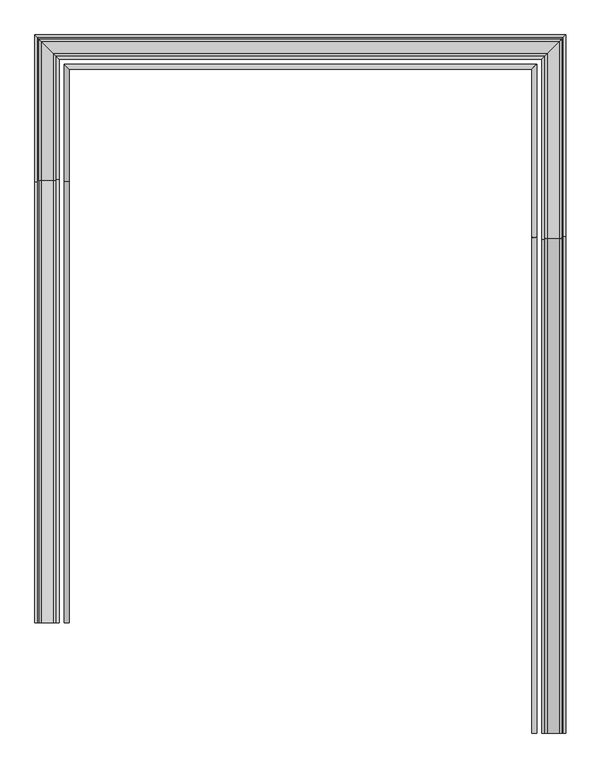
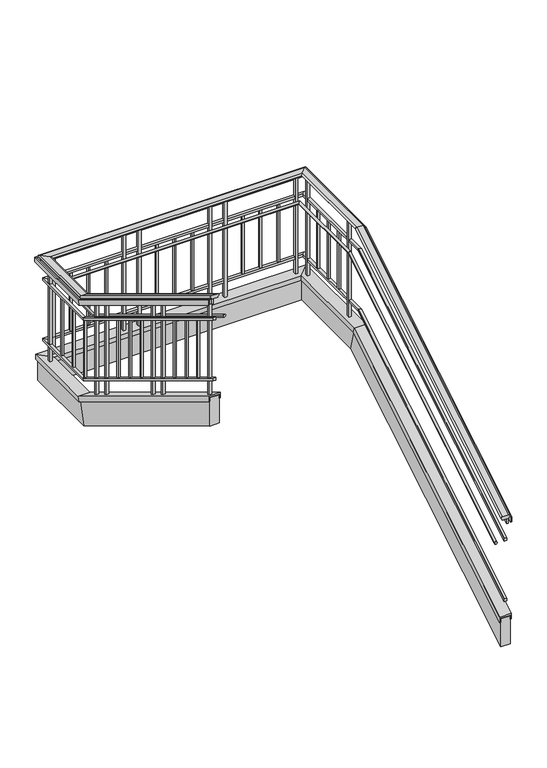
"""IFC4 building model written with IfcOpenShell, lengths in millimetres: railing geometry."""

from ifc_helpers import new_model, si_unit, frame, origin, place, context, project, spatial, polyline, ellipse_curve, outline, extrude, faceted_brep, source, transform, mapped, element, save
from ifc_brep_helpers import plane_surface, cylinder_surface, advanced_brep


def railing_cfa20eb0(model_context):
    return source(origin(), model_context, "Body", "SolidModel", [
        advanced_brep(
        [(-18297.9601205, -2131.266536, 1273.259246), (-18297.9601205, -2131.266536, 1247.2709218), (-18297.9601205, -2131.266536, 1236.1333333), (-18234.6103678, -2131.266536, 1236.1333333), (-18234.6103678, -2131.266536, 1247.1970062), (-18234.6103678, -2131.266536, 1273.259246), (-18297.9601205, 374.4632081, 2791.8833333), (-18297.9601205, 380.6724315, 2769.6581748), (-18297.9601205, 383.333464, 2760.1333333), (-18234.6103678, 383.333464, 2760.1333333), (-18234.6103678, 380.6900917, 2769.5949623), (-18234.6103678, 374.4632081, 2791.8833333), (-18297.9601205, 1312.1712113, 2791.8833333), (-18297.9601205, 1312.1712113, 2769.6581748), (-18297.9601205, 1312.1712113, 2760.1333333), (-18234.6103678, 1375.520964, 2760.1333333), (-18234.6103678, 1375.520964, 2769.5949623), (-18234.6103678, 1375.520964, 2791.8833333), (-20801.9121283, 1312.1712113, 2791.8833333), (-20801.9121283, 1312.1712113, 2769.6581748), (-20801.9121283, 1312.1712113, 2760.1333333), (-20865.2618809, 1375.520964, 2760.1333333), (-20865.2618809, 1375.520964, 2769.5949623), (-20865.2618809, 1375.520964, 2791.8833333), (-20801.9121283, 671.6037198, 2791.8833333), (-20801.9121283, 665.3944964, 2769.6581748), (-20801.9121283, 662.733464, 2760.1333333), (-20865.2618809, 662.733464, 2760.1333333), (-20865.2618809, 665.3768362, 2769.5949623), (-20865.2618809, 671.6037198, 2791.8833333), (-20801.9121283, -1572.466536, 4151.9259127), (-20865.2618809, -1572.466536, 4151.9259127), (-20865.2618809, -1572.466536, 4125.8636728), (-20865.2618809, -1572.466536, 4114.8), (-20801.9121283, -1572.466536, 4114.8), (-20801.9121283, -1572.466536, 4125.9375884)],
        [
            (0, 1, ellipse_curve(frame((-18297.9601205, -2131.266536, 1260.2650839), z_axis=(0.0, -1.0, 0.0), x_axis=(0.0, 0.0, -1.0)), 12.9941621, 11.1125793)),
            (1, 2),
            (2, 3),
            (3, 4),
            (4, 5, ellipse_curve(frame((-18234.6103678, -2131.266536, 1260.2281261), z_axis=(0.0, -1.0, 0.0), x_axis=(0.0, 0.0, -1.0)), 13.0311199, 11.1441855)),
            (5, 0),
            (0, 6),
            (6, 7, ellipse_curve(frame((-18297.9601205, 377.5678198, 2780.7707541), z_axis=(0.0, -0.9631193673564087, -0.26907449567543734), x_axis=(0.0, 0.2690744956754369, -0.9631193673564088)), 11.5381121, 11.1125793)),
            (7, 1),
            (7, 8),
            (8, 2),
            (8, 9),
            (9, 3),
            (9, 10),
            (10, 4),
            (10, 11, ellipse_curve(frame((-18234.6103678, 377.5766499, 2780.7391478), z_axis=(0.0, -0.9631193673564087, -0.26907449567543734), x_axis=(0.0, 0.2690744956754369, -0.9631193673564088)), 11.5709287, 11.1441855)),
            (11, 5),
            (11, 6),
            (6, 12),
            (12, 13, ellipse_curve(frame((-18297.9601205, 1312.1712113, 2780.7707541), z_axis=(0.7071067811865475, -0.7071067811865475, 0.0), x_axis=(-0.7071067811865474, -0.7071067811865476, 0.0)), 15.7155603, 11.1125793)),
            (13, 7),
            (13, 14),
            (14, 8),
            (14, 15),
            (15, 9),
            (15, 16),
            (16, 10),
            (16, 17, ellipse_curve(frame((-18234.6103678, 1375.520964, 2780.7391478), z_axis=(0.7071067811865475, -0.7071067811865475, 0.0), x_axis=(-0.7071067811865474, -0.7071067811865476, 0.0)), 15.7602583, 11.1441855)),
            (17, 11),
            (17, 12),
            (12, 18),
            (18, 19, ellipse_curve(frame((-20801.9121283, 1312.1712113, 2780.7707541), z_axis=(0.7071067811865475, 0.7071067811865475, 0.0), x_axis=(0.7071067811865476, -0.7071067811865474, 0.0)), 15.7155603, 11.1125793)),
            (19, 13),
            (19, 20),
            (20, 14),
            (20, 21),
            (21, 15),
            (21, 22),
            (22, 16),
            (22, 23, ellipse_curve(frame((-20865.2618809, 1375.520964, 2780.7391478), z_axis=(0.7071067811865475, 0.7071067811865475, 0.0), x_axis=(0.7071067811865476, -0.7071067811865474, 0.0)), 15.7602583, 11.1441855)),
            (23, 17),
            (23, 18),
            (18, 24),
            (24, 25, ellipse_curve(frame((-20801.9121283, 668.4991081, 2780.7707541), z_axis=(0.0, 0.9631193673564087, -0.2690744956754374), x_axis=(0.0, 0.26907449567543773, 0.9631193673564086)), 11.5381121, 11.1125793)),
            (25, 19),
            (25, 26),
            (26, 20),
            (26, 27),
            (27, 21),
            (27, 28),
            (28, 22),
            (28, 29, ellipse_curve(frame((-20865.2618809, 668.490278, 2780.7391478), z_axis=(0.0, 0.9631193673564087, -0.2690744956754374), x_axis=(0.0, 0.26907449567543773, 0.9631193673564086)), 11.5709287, 11.1441855)),
            (29, 23),
            (29, 24),
            (30, 31),
            (31, 32, ellipse_curve(frame((-20865.2618809, -1572.466536, 4138.8947927), z_axis=(0.0, -1.0, 0.0), x_axis=(0.0, 0.0, -1.0)), 13.0311199, 11.1441855)),
            (32, 33),
            (33, 34),
            (34, 35),
            (35, 30, ellipse_curve(frame((-20801.9121283, -1572.466536, 4138.9317505), z_axis=(0.0, -1.0, 0.0), x_axis=(0.0, 0.0, -1.0)), 12.9941621, 11.1125793)),
            (24, 30),
            (35, 25),
            (34, 26),
            (33, 27),
            (32, 28),
            (31, 29),
        ],
        [
            plane_surface(frame((-18266.3603678, -2131.266536, 1236.1333333), z_axis=(0.0, -1.0, 0.0), x_axis=(0.0, 0.0, 1.0))),
            cylinder_surface(frame((-18297.9601205, -2141.9629466, 1253.7824108), z_axis=(0.0, -0.8551978315540181, -0.518301716093344), x_axis=(1.0, 0.0, 0.0)), 11.1125793),
            plane_surface(frame((-18297.9601205, -2131.266536, 1247.2709218), z_axis=(-1.0000000000000002, 0.0, 0.0), x_axis=(0.0, 0.8551978315540182, 0.518301716093344))),
            plane_surface(frame((-18297.9601205, -2131.266536, 1236.1333333), z_axis=(0.0, 0.518301716093344, -0.8551978315540181), x_axis=(0.0, 0.8551978315540181, 0.518301716093344))),
            plane_surface(frame((-18234.6103678, -2131.266536, 1236.1333333), z_axis=(1.0, 0.0, 0.0), x_axis=(0.0, 0.8551978315540181, 0.518301716093344))),
            cylinder_surface(frame((-18234.6103678, -2141.9465651, 1253.7553812), z_axis=(0.0, -0.8551978315540181, -0.518301716093344), x_axis=(1.0, 0.0, 0.0)), 11.1441855),
            plane_surface(frame((-18234.6103678, -2131.266536, 1273.259246), z_axis=(0.0, -0.518301716093344, 0.8551978315540181), x_axis=(0.0, 0.8551978315540181, 0.518301716093344))),
            cylinder_surface(frame((-18297.9601205, 383.333464, 2780.7707541), z_axis=(0.0, -1.0, 0.0), x_axis=(1.0, 0.0, 0.0)), 11.1125793),
            plane_surface(frame((-18297.9601205, 380.6724315, 2769.6581748), z_axis=(-1.0, 0.0, 0.0), x_axis=(0.0, 1.0, 0.0))),
            plane_surface(frame((-18297.9601205, 383.333464, 2760.1333333), z_axis=(0.0, 0.0, -1.0), x_axis=(0.0, 1.0, 0.0))),
            plane_surface(frame((-18234.6103678, 383.333464, 2760.1333333), z_axis=(1.0, 0.0, 0.0), x_axis=(0.0, 1.0, 0.0))),
            cylinder_surface(frame((-18234.6103678, 383.333464, 2780.7391478), z_axis=(0.0, -1.0, 0.0), x_axis=(1.0, 0.0, 0.0)), 11.1441855),
            plane_surface(frame((-18234.6103678, 374.4632081, 2791.8833333), z_axis=(0.0, 0.0, 1.0), x_axis=(0.0, 1.0, 0.0))),
            cylinder_surface(frame((-18266.3603678, 1312.1712113, 2780.7707541), z_axis=(1.0, 0.0, 0.0), x_axis=(0.0, 1.0, 0.0)), 11.1125793),
            plane_surface(frame((-18297.9601205, 1312.1712113, 2769.6581748), z_axis=(0.0, -1.0, 0.0), x_axis=(-1.0, 0.0, 0.0))),
            plane_surface(frame((-18297.9601205, 1312.1712113, 2760.1333333), z_axis=(0.0, 0.0, -1.0), x_axis=(-1.0, 0.0, 0.0))),
            plane_surface(frame((-18234.6103678, 1375.520964, 2760.1333333), z_axis=(0.0, 1.0, 0.0), x_axis=(-1.0, 0.0, 0.0))),
            cylinder_surface(frame((-18266.3603678, 1375.520964, 2780.7391478), z_axis=(1.0, 0.0, 0.0), x_axis=(0.0, 1.0, 0.0)), 11.1441855),
            plane_surface(frame((-18234.6103678, 1375.520964, 2791.8833333), z_axis=(0.0, 0.0, 1.0), x_axis=(-1.0, 0.0, 0.0))),
            cylinder_surface(frame((-20801.9121283, 1343.770964, 2780.7707541), z_axis=(0.0, 1.0, 0.0), x_axis=(-1.0, 0.0, 0.0)), 11.1125793),
            plane_surface(frame((-20801.9121283, 1312.1712113, 2769.6581748), z_axis=(1.0, 0.0, 0.0), x_axis=(0.0, -1.0, 0.0))),
            plane_surface(frame((-20801.9121283, 1312.1712113, 2760.1333333), z_axis=(0.0, 0.0, -1.0), x_axis=(0.0, -1.0, 0.0))),
            plane_surface(frame((-20865.2618809, 1375.520964, 2760.1333333), z_axis=(-1.0, 0.0, 0.0), x_axis=(0.0, -1.0, 0.0))),
            cylinder_surface(frame((-20865.2618809, 1343.770964, 2780.7391478), z_axis=(0.0, 1.0, 0.0), x_axis=(-1.0, 0.0, 0.0)), 11.1441855),
            plane_surface(frame((-20865.2618809, 1375.520964, 2791.8833333), z_axis=(0.0, 0.0, 1.0), x_axis=(0.0, -1.0, 0.0))),
            plane_surface(frame((-20833.5118809, -1572.466536, 4114.8), z_axis=(0.0, -1.0, 0.0), x_axis=(0.0, 0.0, -1.0))),
            cylinder_surface(frame((-20801.9121283, 673.4298745, 2777.7824108), z_axis=(0.0, 0.855197831554018, -0.5183017160933441), x_axis=(-1.0, 0.0, 0.0)), 11.1125793),
            plane_surface(frame((-20801.9121283, 665.3944964, 2769.6581748), z_axis=(1.0, 0.0, 0.0), x_axis=(0.0, -0.8551978315540181, 0.5183017160933441))),
            plane_surface(frame((-20801.9121283, 662.733464, 2760.1333333), z_axis=(0.0, -0.5183017160933441, -0.855197831554018), x_axis=(0.0, -0.855197831554018, 0.5183017160933441))),
            plane_surface(frame((-20865.2618809, 662.733464, 2760.1333333), z_axis=(-1.0000000000000002, 0.0, 0.0), x_axis=(0.0, -0.8551978315540181, 0.5183017160933442))),
            cylinder_surface(frame((-20865.2618809, 673.413493, 2777.7553812), z_axis=(0.0, 0.855197831554018, -0.5183017160933441), x_axis=(-1.0, 0.0, 0.0)), 11.1441855),
            plane_surface(frame((-20865.2618809, 671.6037198, 2791.8833333), z_axis=(0.0, 0.5183017160933441, 0.8551978315540181), x_axis=(0.0, -0.8551978315540181, 0.5183017160933441))),
        ],
        [
            (0, [[1, 2, 3, 4, 5, 6]]),
            (1, [[-1, 7, 8, 9]]),
            (2, [[-2, -9, 10, 11]]),
            (3, [[-3, -11, 12, 13]]),
            (4, [[-4, -13, 14, 15]]),
            (5, [[-5, -15, 16, 17]]),
            (6, [[-6, -17, 18, -7]]),
            (7, [[-8, 19, 20, 21]]),
            (8, [[-10, -21, 22, 23]]),
            (9, [[-12, -23, 24, 25]]),
            (10, [[-14, -25, 26, 27]]),
            (11, [[-16, -27, 28, 29]]),
            (12, [[-18, -29, 30, -19]]),
            (13, [[-20, 31, 32, 33]]),
            (14, [[-22, -33, 34, 35]]),
            (15, [[-24, -35, 36, 37]]),
            (16, [[-26, -37, 38, 39]]),
            (17, [[-28, -39, 40, 41]]),
            (18, [[-30, -41, 42, -31]]),
            (19, [[-32, 43, 44, 45]]),
            (20, [[-34, -45, 46, 47]]),
            (21, [[-36, -47, 48, 49]]),
            (22, [[-38, -49, 50, 51]]),
            (23, [[-40, -51, 52, 53]]),
            (24, [[-42, -53, 54, -43]]),
            (25, [[55, 56, 57, 58, 59, 60]]),
            (26, [[-44, 61, -60, 62]]),
            (27, [[-46, -62, -59, 63]]),
            (28, [[-48, -63, -58, 64]]),
            (29, [[-50, -64, -57, 65]]),
            (30, [[-52, -65, -56, 66]]),
            (31, [[-54, -66, -55, -61]]),
        ],
    ),
        faceted_brep([(-18240.8852442, -2131.266536, 1236.1333333), (-18253.5852442, -2131.266536, 1236.1333333), (-18253.5852442, -2131.266536, 1184.1570556), (-18240.8852442, -2131.266536, 1184.1570556), (-18240.8852442, 383.333464, 2760.1333333), (-18253.5852442, 383.333464, 2760.1333333), (-18253.5852442, 395.7518222, 2715.6833333), (-18240.8852442, 395.7518222, 2715.6833333), (-18240.8852442, 1369.2460876, 2760.1333333), (-18253.5852442, 1356.5460876, 2760.1333333), (-18253.5852442, 1356.5460876, 2715.6833333), (-18240.8852442, 1369.2460876, 2715.6833333), (-20858.9870046, 1369.2460876, 2760.1333333), (-20846.2870046, 1356.5460876, 2760.1333333), (-20846.2870046, 1356.5460876, 2715.6833333), (-20858.9870046, 1369.2460876, 2715.6833333), (-20858.9870046, 662.733464, 2760.1333333), (-20846.2870046, 662.733464, 2760.1333333), (-20846.2870046, 650.3151057, 2715.6833333), (-20858.9870046, 650.3151057, 2715.6833333), (-20858.9870046, -1572.466536, 4114.8), (-20858.9870046, -1572.466536, 4062.8237223), (-20846.2870046, -1572.466536, 4062.8237223), (-20846.2870046, -1572.466536, 4114.8)], [[[0, 1, 2, 3]], [[1, 0, 4, 5]], [[2, 1, 5, 6]], [[3, 2, 6, 7]], [[0, 3, 7, 4]], [[5, 4, 8, 9]], [[6, 5, 9, 10]], [[7, 6, 10, 11]], [[4, 7, 11, 8]], [[9, 8, 12, 13]], [[10, 9, 13, 14]], [[11, 10, 14, 15]], [[8, 11, 15, 12]], [[13, 12, 16, 17]], [[14, 13, 17, 18]], [[15, 14, 18, 19]], [[12, 15, 19, 16]], [[20, 21, 22, 23]], [[17, 16, 20, 23]], [[18, 17, 23, 22]], [[19, 18, 22, 21]], [[16, 19, 21, 20]]]),
        faceted_brep([(-18202.7852442, -2131.266536, 1236.1333333), (-18215.4852442, -2131.266536, 1236.1333333), (-18215.4852442, -2131.266536, 1184.1570556), (-18202.7852442, -2131.266536, 1184.1570556), (-18202.7852442, 383.333464, 2760.1333333), (-18215.4852442, 383.333464, 2760.1333333), (-18215.4852442, 395.7518222, 2715.6833333), (-18202.7852442, 395.7518222, 2715.6833333), (-18202.7852442, 1407.3460876, 2760.1333333), (-18215.4852442, 1394.6460876, 2760.1333333), (-18215.4852442, 1394.6460876, 2715.6833333), (-18202.7852442, 1407.3460876, 2715.6833333), (-20897.0870046, 1407.3460876, 2760.1333333), (-20884.3870046, 1394.6460876, 2760.1333333), (-20884.3870046, 1394.6460876, 2715.6833333), (-20897.0870046, 1407.3460876, 2715.6833333), (-20897.0870046, 662.733464, 2760.1333333), (-20884.3870046, 662.733464, 2760.1333333), (-20884.3870046, 650.3151057, 2715.6833333), (-20897.0870046, 650.3151057, 2715.6833333), (-20897.0870046, -1572.466536, 4114.8), (-20897.0870046, -1572.466536, 4062.8237223), (-20884.3870046, -1572.466536, 4062.8237223), (-20884.3870046, -1572.466536, 4114.8)], [[[0, 1, 2, 3]], [[1, 0, 4, 5]], [[2, 1, 5, 6]], [[3, 2, 6, 7]], [[0, 3, 7, 4]], [[5, 4, 8, 9]], [[6, 5, 9, 10]], [[7, 6, 10, 11]], [[4, 7, 11, 8]], [[9, 8, 12, 13]], [[10, 9, 13, 14]], [[11, 10, 14, 15]], [[8, 11, 15, 12]], [[13, 12, 16, 17]], [[14, 13, 17, 18]], [[15, 14, 18, 19]], [[12, 15, 19, 16]], [[20, 21, 22, 23]], [[17, 16, 20, 23]], [[18, 17, 23, 22]], [[19, 18, 22, 21]], [[16, 19, 21, 20]]]),
        faceted_brep([(-18253.6603678, -2131.266536, 1037.2340635), (-18279.0603678, -2131.266536, 1037.2340635), (-18279.0603678, -2131.266536, 1007.5333333), (-18253.6603678, -2131.266536, 1007.5333333), (-18253.6603678, 376.2372592, 2556.9333333), (-18279.0603678, 376.2372592, 2556.9333333), (-18279.0603678, 383.333464, 2531.5333333), (-18253.6603678, 383.333464, 2531.5333333), (-18253.6603678, 1356.470964, 2556.9333333), (-18279.0603678, 1331.070964, 2556.9333333), (-18279.0603678, 1331.070964, 2531.5333333), (-18253.6603678, 1356.470964, 2531.5333333), (-20846.2118809, 1356.470964, 2556.9333333), (-20820.8118809, 1331.070964, 2556.9333333), (-20820.8118809, 1331.070964, 2531.5333333), (-20846.2118809, 1356.470964, 2531.5333333), (-20846.2118809, 669.8296687, 2556.9333333), (-20820.8118809, 669.8296687, 2556.9333333), (-20820.8118809, 662.733464, 2531.5333333), (-20846.2118809, 662.733464, 2531.5333333), (-20846.2118809, -1572.466536, 3915.9007301), (-20846.2118809, -1572.466536, 3886.2), (-20820.8118809, -1572.466536, 3886.2), (-20820.8118809, -1572.466536, 3915.9007301)], [[[0, 1, 2, 3]], [[1, 0, 4, 5]], [[2, 1, 5, 6]], [[3, 2, 6, 7]], [[0, 3, 7, 4]], [[5, 4, 8, 9]], [[6, 5, 9, 10]], [[7, 6, 10, 11]], [[4, 7, 11, 8]], [[9, 8, 12, 13]], [[10, 9, 13, 14]], [[11, 10, 14, 15]], [[8, 11, 15, 12]], [[13, 12, 16, 17]], [[14, 13, 17, 18]], [[15, 14, 18, 19]], [[12, 15, 19, 16]], [[20, 21, 22, 23]], [[17, 16, 20, 23]], [[18, 17, 23, 22]], [[19, 18, 22, 21]], [[16, 19, 21, 20]]]),
        advanced_brep(
        [(-18375.8978678, -2131.266536, 1020.2333333), (-18350.4978678, -2131.266536, 1020.2333333), (-18375.8978678, 383.333464, 2544.2333333), (-18350.4978678, 383.333464, 2544.2333333), (-18375.8978678, 1234.233464, 2544.2333333), (-18350.4978678, 1259.633464, 2544.2333333), (-20723.9743809, 1234.233464, 2544.2333333), (-20749.3743809, 1259.633464, 2544.2333333), (-20723.9743809, 662.733464, 2544.2333333), (-20749.3743809, 662.733464, 2544.2333333), (-20723.9743809, -1572.466536, 3898.9), (-20749.3743809, -1572.466536, 3898.9)],
        [
            (0, 1, ellipse_curve(frame((-18363.1978678, -2131.266536, 1020.2333333), z_axis=(0.0, -1.0, 0.0), x_axis=(0.0, 0.0, -1.0)), 14.8503651, 12.7)),
            (1, 0, ellipse_curve(frame((-18363.1978678, -2131.266536, 1020.2333333), z_axis=(0.0, -1.0, 0.0), x_axis=(0.0, 0.0, -1.0)), 14.8503651, 12.7)),
            (0, 2),
            (2, 3, ellipse_curve(frame((-18363.1978678, 383.333464, 2544.2333333), z_axis=(0.0, -0.9631193673564087, -0.2690744956754374), x_axis=(0.0, 0.2690744956754374, -0.9631193673564086)), 13.1863198, 12.7)),
            (3, 1),
            (3, 2, ellipse_curve(frame((-18363.1978678, 383.333464, 2544.2333333), z_axis=(0.0, -0.9631193673564087, -0.2690744956754374), x_axis=(0.0, 0.2690744956754374, -0.9631193673564086)), 13.1863198, 12.7)),
            (2, 4),
            (4, 5, ellipse_curve(frame((-18363.1978678, 1246.933464, 2544.2333333), z_axis=(0.7071067811865475, -0.7071067811865475, 0.0), x_axis=(-0.7071067811865474, -0.7071067811865476, 0.0)), 17.9605122, 12.7)),
            (5, 3),
            (5, 4, ellipse_curve(frame((-18363.1978678, 1246.933464, 2544.2333333), z_axis=(0.7071067811865475, -0.7071067811865475, 0.0), x_axis=(-0.7071067811865474, -0.7071067811865476, 0.0)), 17.9605122, 12.7)),
            (4, 6),
            (6, 7, ellipse_curve(frame((-20736.6743809, 1246.933464, 2544.2333333), z_axis=(0.7071067811865475, 0.7071067811865475, 0.0), x_axis=(0.7071067811865476, -0.7071067811865474, 0.0)), 17.9605122, 12.7)),
            (7, 5),
            (7, 6, ellipse_curve(frame((-20736.6743809, 1246.933464, 2544.2333333), z_axis=(0.7071067811865475, 0.7071067811865475, 0.0), x_axis=(0.7071067811865476, -0.7071067811865474, 0.0)), 17.9605122, 12.7)),
            (6, 8),
            (8, 9, ellipse_curve(frame((-20736.6743809, 662.733464, 2544.2333333), z_axis=(0.0, 0.9631193673564087, -0.26907449567543756), x_axis=(0.0, 0.26907449567543773, 0.9631193673564087)), 13.1863198, 12.7)),
            (9, 7),
            (9, 8, ellipse_curve(frame((-20736.6743809, 662.733464, 2544.2333333), z_axis=(0.0, 0.9631193673564087, -0.26907449567543756), x_axis=(0.0, 0.26907449567543773, 0.9631193673564087)), 13.1863198, 12.7)),
            (10, 11, ellipse_curve(frame((-20736.6743809, -1572.466536, 3898.9), z_axis=(0.0, -1.0, 0.0), x_axis=(0.0, 0.0, -1.0)), 14.8503651, 12.7)),
            (11, 10, ellipse_curve(frame((-20736.6743809, -1572.466536, 3898.9), z_axis=(0.0, -1.0, 0.0), x_axis=(0.0, 0.0, -1.0)), 14.8503651, 12.7)),
            (8, 10),
            (11, 9),
        ],
        [
            plane_surface(frame((-18363.1978678, -2131.266536, 1020.2333333), z_axis=(0.0, -1.0, 0.0), x_axis=(0.0, 0.0, 1.0))),
            cylinder_surface(frame((-18363.1978678, -2131.266536, 1020.2333333), z_axis=(0.0, -0.8551978315540182, -0.518301716093344), x_axis=(1.0, 0.0, 0.0)), 12.7),
            cylinder_surface(frame((-18363.1978678, 383.333464, 2544.2333333), z_axis=(0.0, -1.0, 0.0), x_axis=(1.0, 0.0, 0.0)), 12.7),
            cylinder_surface(frame((-18363.1978678, 1246.933464, 2544.2333333), z_axis=(1.0, 0.0, 0.0), x_axis=(0.0, 1.0, 0.0)), 12.7),
            cylinder_surface(frame((-20736.6743809, 1246.933464, 2544.2333333), z_axis=(0.0, 1.0, 0.0), x_axis=(-1.0, 0.0, 0.0)), 12.7),
            plane_surface(frame((-20736.6743809, -1572.466536, 3898.9), z_axis=(0.0, -1.0, 0.0), x_axis=(0.0, 0.0, -1.0))),
            cylinder_surface(frame((-20736.6743809, 662.733464, 2544.2333333), z_axis=(0.0, 0.855197831554018, -0.5183017160933443), x_axis=(-1.0, 0.0, 0.0)), 12.7),
        ],
        [
            (0, [[1, 2]]),
            (1, [[-1, 3, 4, 5]]),
            (1, [[-2, -5, 6, -3]]),
            (2, [[-4, 7, 8, 9]]),
            (2, [[-6, -9, 10, -7]]),
            (3, [[-8, 11, 12, 13]]),
            (3, [[-10, -13, 14, -11]]),
            (4, [[-12, 15, 16, 17]]),
            (4, [[-14, -17, 18, -15]]),
            (5, [[19, 20]]),
            (6, [[-16, 21, -20, 22]]),
            (6, [[-18, -22, -19, -21]]),
        ],
    ),
        faceted_brep([(-18253.6603678, -2131.266536, 402.2340635), (-18279.0603678, -2131.266536, 402.2340635), (-18279.0603678, -2131.266536, 372.5333333), (-18253.6603678, -2131.266536, 372.5333333), (-18253.6603678, 376.2372592, 1921.9333333), (-18279.0603678, 376.2372592, 1921.9333333), (-18279.0603678, 383.333464, 1896.5333333), (-18253.6603678, 383.333464, 1896.5333333), (-18253.6603678, 1356.470964, 1921.9333333), (-18279.0603678, 1331.070964, 1921.9333333), (-18279.0603678, 1331.070964, 1896.5333333), (-18253.6603678, 1356.470964, 1896.5333333), (-20846.2118809, 1356.470964, 1921.9333333), (-20820.8118809, 1331.070964, 1921.9333333), (-20820.8118809, 1331.070964, 1896.5333333), (-20846.2118809, 1356.470964, 1896.5333333), (-20846.2118809, 669.8296687, 1921.9333333), (-20820.8118809, 669.8296687, 1921.9333333), (-20820.8118809, 662.733464, 1896.5333333), (-20846.2118809, 662.733464, 1896.5333333), (-20846.2118809, -1572.466536, 3280.9007301), (-20846.2118809, -1572.466536, 3251.2), (-20820.8118809, -1572.466536, 3251.2), (-20820.8118809, -1572.466536, 3280.9007301)], [[[0, 1, 2, 3]], [[1, 0, 4, 5]], [[2, 1, 5, 6]], [[3, 2, 6, 7]], [[0, 3, 7, 4]], [[5, 4, 8, 9]], [[6, 5, 9, 10]], [[7, 6, 10, 11]], [[4, 7, 11, 8]], [[9, 8, 12, 13]], [[10, 9, 13, 14]], [[11, 10, 14, 15]], [[8, 11, 15, 12]], [[13, 12, 16, 17]], [[14, 13, 17, 18]], [[15, 14, 18, 19]], [[12, 15, 19, 16]], [[20, 21, 22, 23]], [[17, 16, 20, 23]], [[18, 17, 23, 22]], [[19, 18, 22, 21]], [[16, 19, 21, 20]]]),
        faceted_brep([(-18325.0227442, -2131.266536, 226.6724478), (-18325.0227442, -2131.266536, 169.3333333), (-18312.3227442, -2131.266536, 169.3333333), (-18312.3227442, -2131.266536, 211.8220828), (-18220.2477442, -2131.266536, 211.8220828), (-18220.2477442, -2131.266536, 169.3333333), (-18207.5477442, -2131.266536, 169.3333333), (-18207.5477442, -2131.266536, 226.6724478), (-18325.0227442, 369.6337976, 1742.3696197), (-18325.0227442, 383.333464, 1693.3333333), (-18312.3227442, 383.333464, 1693.3333333), (-18312.3227442, 373.1818999, 1729.6696197), (-18220.2477442, 373.1818999, 1729.6696197), (-18220.2477442, 383.333464, 1693.3333333), (-18207.5477442, 383.333464, 1693.3333333), (-18207.5477442, 369.6337976, 1742.3696197), (-18325.0227442, 1285.1085876, 1742.3696197), (-18325.0227442, 1285.1085876, 1693.3333333), (-18312.3227442, 1297.8085876, 1693.3333333), (-18312.3227442, 1297.8085876, 1729.6696197), (-18220.2477442, 1389.8835876, 1729.6696197), (-18220.2477442, 1389.8835876, 1693.3333333), (-18207.5477442, 1402.5835876, 1693.3333333), (-18207.5477442, 1402.5835876, 1742.3696197), (-20774.8495046, 1285.1085876, 1742.3696197), (-20774.8495046, 1285.1085876, 1693.3333333), (-20787.5495046, 1297.8085876, 1693.3333333), (-20787.5495046, 1297.8085876, 1729.6696197), (-20879.6245046, 1389.8835876, 1729.6696197), (-20879.6245046, 1389.8835876, 1693.3333333), (-20892.3245046, 1402.5835876, 1693.3333333), (-20892.3245046, 1402.5835876, 1742.3696197), (-20774.8495046, 676.4331303, 1742.3696197), (-20774.8495046, 662.733464, 1693.3333333), (-20787.5495046, 662.733464, 1693.3333333), (-20787.5495046, 672.885028, 1729.6696197), (-20879.6245046, 672.885028, 1729.6696197), (-20879.6245046, 662.733464, 1693.3333333), (-20892.3245046, 662.733464, 1693.3333333), (-20892.3245046, 676.4331303, 1742.3696197), (-20774.8495046, -1572.466536, 3105.3391145), (-20892.3245046, -1572.466536, 3105.3391145), (-20892.3245046, -1572.466536, 3048.0), (-20879.6245046, -1572.466536, 3048.0), (-20879.6245046, -1572.466536, 3090.4887494), (-20787.5495046, -1572.466536, 3090.4887494), (-20787.5495046, -1572.466536, 3048.0), (-20774.8495046, -1572.466536, 3048.0)], [[[0, 1, 2, 3, 4, 5, 6, 7]], [[1, 0, 8, 9]], [[2, 1, 9, 10]], [[3, 2, 10, 11]], [[4, 3, 11, 12]], [[5, 4, 12, 13]], [[6, 5, 13, 14]], [[7, 6, 14, 15]], [[0, 7, 15, 8]], [[9, 8, 16, 17]], [[10, 9, 17, 18]], [[11, 10, 18, 19]], [[12, 11, 19, 20]], [[13, 12, 20, 21]], [[14, 13, 21, 22]], [[15, 14, 22, 23]], [[8, 15, 23, 16]], [[17, 16, 24, 25]], [[18, 17, 25, 26]], [[19, 18, 26, 27]], [[20, 19, 27, 28]], [[21, 20, 28, 29]], [[22, 21, 29, 30]], [[23, 22, 30, 31]], [[16, 23, 31, 24]], [[25, 24, 32, 33]], [[26, 25, 33, 34]], [[27, 26, 34, 35]], [[28, 27, 35, 36]], [[29, 28, 36, 37]], [[30, 29, 37, 38]], [[31, 30, 38, 39]], [[24, 31, 39, 32]], [[40, 41, 42, 43, 44, 45, 46, 47]], [[33, 32, 40, 47]], [[34, 33, 47, 46]], [[35, 34, 46, 45]], [[36, 35, 45, 44]], [[37, 36, 44, 43]], [[38, 37, 43, 42]], [[39, 38, 42, 41]], [[32, 39, 41, 40]]]),
        faceted_brep([(-18312.3227442, -2131.266536, 207.5213526), (-18312.3227442, -2131.266536, -89.4859486), (-18220.2477442, -2131.266536, -89.4859486), (-18220.2477442, -2131.266536, 207.5213526), (-18312.3227442, 380.2781046, 1729.6696197), (-18312.3227442, 451.2401517, 1475.6696197), (-18220.2477442, 451.2401517, 1475.6696197), (-18220.2477442, 380.2781046, 1729.6696197), (-18312.3227442, 1297.8085876, 1729.6696197), (-18312.3227442, 1297.8085876, 1475.6696197), (-18220.2477442, 1389.8835876, 1475.6696197), (-18220.2477442, 1389.8835876, 1729.6696197), (-20787.5495046, 1297.8085876, 1729.6696197), (-20787.5495046, 1297.8085876, 1475.6696197), (-20879.6245046, 1389.8835876, 1475.6696197), (-20879.6245046, 1389.8835876, 1729.6696197), (-20787.5495046, 665.7888233, 1729.6696197), (-20787.5495046, 594.8267762, 1475.6696197), (-20879.6245046, 594.8267762, 1475.6696197), (-20879.6245046, 665.7888233, 1729.6696197), (-20787.5495046, -1572.466536, 3086.1880193), (-20879.6245046, -1572.466536, 3086.1880193), (-20879.6245046, -1572.466536, 2789.180718), (-20787.5495046, -1572.466536, 2789.180718)], [[[0, 1, 2, 3]], [[1, 0, 4, 5]], [[2, 1, 5, 6]], [[3, 2, 6, 7]], [[0, 3, 7, 4]], [[5, 4, 8, 9]], [[6, 5, 9, 10]], [[7, 6, 10, 11]], [[4, 7, 11, 8]], [[9, 8, 12, 13]], [[10, 9, 13, 14]], [[11, 10, 14, 15]], [[8, 11, 15, 12]], [[13, 12, 16, 17]], [[14, 13, 17, 18]], [[15, 14, 18, 19]], [[12, 15, 19, 16]], [[20, 21, 22, 23]], [[17, 16, 20, 23]], [[18, 17, 23, 22]], [[19, 18, 22, 21]], [[16, 19, 21, 20]]]),
        extrude(outline(polyline([(-20843.4337559, -1474.0765544), (-20818.0337559, -1474.0765544), (-20818.0337559, -1499.4765544), (-20843.4337559, -1499.4765544), (-20843.4337559, -1474.0765544)])), frame((0.0, 0.0, 2987.7356246), z_axis=(0.0, 0.0, 1.0), x_axis=(1.0, 0.0, 0.0)), (0.0, 0.0, 1.0), 1075.1310532),
        extrude(outline(polyline([(-20840.2587559, -1277.308264), (-20821.2087559, -1277.308264), (-20821.2087559, -1296.358264), (-20840.2587559, -1296.358264), (-20840.2587559, -1277.308264)])), frame((0.0, 0.0, 3107.7896562), z_axis=(0.0, 0.0, 1.0), x_axis=(1.0, 0.0, 0.0)), (0.0, 0.0, 1.0), 605.2992699),
        extrude(outline(polyline([(-20840.2587559, -1077.3649735), (-20821.2087559, -1077.3649735), (-20821.2087559, -1096.4149735), (-20840.2587559, -1096.4149735), (-20840.2587559, -1077.3649735)])), frame((0.0, 0.0, 2986.6119044), z_axis=(0.0, 0.0, 1.0), x_axis=(1.0, 0.0, 0.0)), (0.0, 0.0, 1.0), 605.2992699),
        extrude(outline(polyline([(-20840.2587559, -877.4216831), (-20821.2087559, -877.4216831), (-20821.2087559, -896.4716831), (-20840.2587559, -896.4716831), (-20840.2587559, -877.4216831)])), frame((0.0, 0.0, 2865.4341526), z_axis=(0.0, 0.0, 1.0), x_axis=(1.0, 0.0, 0.0)), (0.0, 0.0, 1.0), 605.2992699),
        extrude(outline(polyline([(-20843.4337559, -674.3033927), (-20818.0337559, -674.3033927), (-20818.0337559, -699.7033927), (-20843.4337559, -699.7033927), (-20843.4337559, -674.3033927)])), frame((0.0, 0.0, 2503.0246174), z_axis=(0.0, 0.0, 1.0), x_axis=(1.0, 0.0, 0.0)), (0.0, 0.0, 1.0), 1075.1310532),
        extrude(outline(polyline([(-20843.4337559, -502.9234294), (-20818.0337559, -502.9234294), (-20818.0337559, -528.3234294), (-20843.4337559, -528.3234294), (-20843.4337559, -502.9234294)])), frame((0.0, 0.0, 2399.157973), z_axis=(0.0, 0.0, 1.0), x_axis=(1.0, 0.0, 0.0)), (0.0, 0.0, 1.0), 1075.1310532),
        extrude(outline(polyline([(-20840.2587559, -306.155139), (-20821.2087559, -306.155139), (-20821.2087559, -325.205139), (-20840.2587559, -325.205139), (-20840.2587559, -306.155139)])), frame((0.0, 0.0, 2519.2120046), z_axis=(0.0, 0.0, 1.0), x_axis=(1.0, 0.0, 0.0)), (0.0, 0.0, 1.0), 605.2992699),
        extrude(outline(polyline([(-20840.2587559, -106.2118485), (-20821.2087559, -106.2118485), (-20821.2087559, -125.2618485), (-20840.2587559, -125.2618485), (-20840.2587559, -106.2118485)])), frame((0.0, 0.0, 2398.0342529), z_axis=(0.0, 0.0, 1.0), x_axis=(1.0, 0.0, 0.0)), (0.0, 0.0, 1.0), 605.2992699),
        extrude(outline(polyline([(-20840.2587559, 93.7314419), (-20821.2087559, 93.7314419), (-20821.2087559, 74.6814419), (-20840.2587559, 74.6814419), (-20840.2587559, 93.7314419)])), frame((0.0, 0.0, 2276.8565011), z_axis=(0.0, 0.0, 1.0), x_axis=(1.0, 0.0, 0.0)), (0.0, 0.0, 1.0), 605.2992699),
        extrude(outline(polyline([(-20843.4337559, 296.8497323), (-20818.0337559, 296.8497323), (-20818.0337559, 271.4497323), (-20843.4337559, 271.4497323), (-20843.4337559, 296.8497323)])), frame((0.0, 0.0, 1914.4469659), z_axis=(0.0, 0.0, 1.0), x_axis=(1.0, 0.0, 0.0)), (0.0, 0.0, 1.0), 1075.1310532),
        extrude(outline(polyline([(-20843.4337559, 468.2296956), (-20818.0337559, 468.2296956), (-20818.0337559, 442.8296956), (-20843.4337559, 442.8296956), (-20843.4337559, 468.2296956)])), frame((0.0, 0.0, 1810.5803215), z_axis=(0.0, 0.0, 1.0), x_axis=(1.0, 0.0, 0.0)), (0.0, 0.0, 1.0), 1075.1310532),
        extrude(outline(polyline([(-20840.2587559, 664.997986), (-20821.2087559, 664.997986), (-20821.2087559, 645.947986), (-20840.2587559, 645.947986), (-20840.2587559, 664.997986)])), frame((0.0, 0.0, 1930.6343531), z_axis=(0.0, 0.0, 1.0), x_axis=(1.0, 0.0, 0.0)), (0.0, 0.0, 1.0), 605.2992699),
        extrude(outline(polyline([(-20840.2587559, 864.9412765), (-20821.2087559, 864.9412765), (-20821.2087559, 845.8912765), (-20840.2587559, 845.8912765), (-20840.2587559, 864.9412765)])), frame((0.0, 0.0, 1921.9333333), z_axis=(0.0, 0.0, 1.0), x_axis=(1.0, 0.0, 0.0)), (0.0, 0.0, 1.0), 609.6),
        extrude(outline(polyline([(-20840.2587559, 1064.8845669), (-20821.2087559, 1064.8845669), (-20821.2087559, 1045.8345669), (-20840.2587559, 1045.8345669), (-20840.2587559, 1064.8845669)])), frame((0.0, 0.0, 1921.9333333), z_axis=(0.0, 0.0, 1.0), x_axis=(1.0, 0.0, 0.0)), (0.0, 0.0, 1.0), 609.6),
        extrude(outline(polyline([(-20843.4337559, 1268.0028573), (-20818.0337559, 1268.0028573), (-20818.0337559, 1242.6028573), (-20843.4337559, 1242.6028573), (-20843.4337559, 1268.0028573)])), frame((0.0, 0.0, 1695.7303208), z_axis=(0.0, 0.0, 1.0), x_axis=(1.0, 0.0, 0.0)), (0.0, 0.0, 1.0), 1064.4030125),
        extrude(outline(polyline([(-20742.6927188, 1353.692839), (-20742.6927188, 1328.292839), (-20768.0927188, 1328.292839), (-20768.0927188, 1353.692839), (-20742.6927188, 1353.692839)])), frame((0.0, 0.0, 1695.7303208), z_axis=(0.0, 0.0, 1.0), x_axis=(1.0, 0.0, 0.0)), (0.0, 0.0, 1.0), 1064.4030125),
        extrude(outline(polyline([(-20570.0719654, 1350.517839), (-20570.0719654, 1331.467839), (-20589.1219654, 1331.467839), (-20589.1219654, 1350.517839), (-20570.0719654, 1350.517839)])), frame((0.0, 0.0, 1921.9333333), z_axis=(0.0, 0.0, 1.0), x_axis=(1.0, 0.0, 0.0)), (0.0, 0.0, 1.0), 609.6),
        extrude(outline(polyline([(-20394.2762121, 1350.517839), (-20394.2762121, 1331.467839), (-20413.3262121, 1331.467839), (-20413.3262121, 1350.517839), (-20394.2762121, 1350.517839)])), frame((0.0, 0.0, 1921.9333333), z_axis=(0.0, 0.0, 1.0), x_axis=(1.0, 0.0, 0.0)), (0.0, 0.0, 1.0), 609.6),
        extrude(outline(polyline([(-20218.4804587, 1350.517839), (-20218.4804587, 1331.467839), (-20237.5304587, 1331.467839), (-20237.5304587, 1350.517839), (-20218.4804587, 1350.517839)])), frame((0.0, 0.0, 1921.9333333), z_axis=(0.0, 0.0, 1.0), x_axis=(1.0, 0.0, 0.0)), (0.0, 0.0, 1.0), 609.6),
        extrude(outline(polyline([(-20039.5097054, 1353.692839), (-20039.5097054, 1328.292839), (-20064.9097054, 1328.292839), (-20064.9097054, 1353.692839), (-20039.5097054, 1353.692839)])), frame((0.0, 0.0, 1695.7303208), z_axis=(0.0, 0.0, 1.0), x_axis=(1.0, 0.0, 0.0)), (0.0, 0.0, 1.0), 1064.4030125),
        extrude(outline(polyline([(-19888.8276311, 1353.692839), (-19888.8276311, 1328.292839), (-19914.2276311, 1328.292839), (-19914.2276311, 1353.692839), (-19888.8276311, 1353.692839)])), frame((0.0, 0.0, 1695.7303208), z_axis=(0.0, 0.0, 1.0), x_axis=(1.0, 0.0, 0.0)), (0.0, 0.0, 1.0), 1064.4030125),
        extrude(outline(polyline([(-19716.2068777, 1350.517839), (-19716.2068777, 1331.467839), (-19735.2568777, 1331.467839), (-19735.2568777, 1350.517839), (-19716.2068777, 1350.517839)])), frame((0.0, 0.0, 1921.9333333), z_axis=(0.0, 0.0, 1.0), x_axis=(1.0, 0.0, 0.0)), (0.0, 0.0, 1.0), 609.6),
        extrude(outline(polyline([(-19540.4111244, 1350.517839), (-19540.4111244, 1331.467839), (-19559.4611244, 1331.467839), (-19559.4611244, 1350.517839), (-19540.4111244, 1350.517839)])), frame((0.0, 0.0, 1921.9333333), z_axis=(0.0, 0.0, 1.0), x_axis=(1.0, 0.0, 0.0)), (0.0, 0.0, 1.0), 609.6),
        extrude(outline(polyline([(-19364.615371, 1350.517839), (-19364.615371, 1331.467839), (-19383.665371, 1331.467839), (-19383.665371, 1350.517839), (-19364.615371, 1350.517839)])), frame((0.0, 0.0, 1921.9333333), z_axis=(0.0, 0.0, 1.0), x_axis=(1.0, 0.0, 0.0)), (0.0, 0.0, 1.0), 609.6),
        extrude(outline(polyline([(-19185.6446177, 1353.692839), (-19185.6446177, 1328.292839), (-19211.0446177, 1328.292839), (-19211.0446177, 1353.692839), (-19185.6446177, 1353.692839)])), frame((0.0, 0.0, 1695.7303208), z_axis=(0.0, 0.0, 1.0), x_axis=(1.0, 0.0, 0.0)), (0.0, 0.0, 1.0), 1064.4030125),
        extrude(outline(polyline([(-19034.9625434, 1353.692839), (-19034.9625434, 1328.292839), (-19060.3625434, 1328.292839), (-19060.3625434, 1353.692839), (-19034.9625434, 1353.692839)])), frame((0.0, 0.0, 1695.7303208), z_axis=(0.0, 0.0, 1.0), x_axis=(1.0, 0.0, 0.0)), (0.0, 0.0, 1.0), 1064.4030125),
        extrude(outline(polyline([(-18862.34179, 1350.517839), (-18862.34179, 1331.467839), (-18881.39179, 1331.467839), (-18881.39179, 1350.517839), (-18862.34179, 1350.517839)])), frame((0.0, 0.0, 1921.9333333), z_axis=(0.0, 0.0, 1.0), x_axis=(1.0, 0.0, 0.0)), (0.0, 0.0, 1.0), 609.6),
        extrude(outline(polyline([(-18686.5460367, 1350.517839), (-18686.5460367, 1331.467839), (-18705.5960367, 1331.467839), (-18705.5960367, 1350.517839), (-18686.5460367, 1350.517839)])), frame((0.0, 0.0, 1921.9333333), z_axis=(0.0, 0.0, 1.0), x_axis=(1.0, 0.0, 0.0)), (0.0, 0.0, 1.0), 609.6),
        extrude(outline(polyline([(-18510.7502833, 1350.517839), (-18510.7502833, 1331.467839), (-18529.8002833, 1331.467839), (-18529.8002833, 1350.517839), (-18510.7502833, 1350.517839)])), frame((0.0, 0.0, 1921.9333333), z_axis=(0.0, 0.0, 1.0), x_axis=(1.0, 0.0, 0.0)), (0.0, 0.0, 1.0), 609.6),
        extrude(outline(polyline([(-18331.77953, 1353.692839), (-18331.77953, 1328.292839), (-18357.17953, 1328.292839), (-18357.17953, 1353.692839), (-18331.77953, 1353.692839)])), frame((0.0, 0.0, 1695.7303208), z_axis=(0.0, 0.0, 1.0), x_axis=(1.0, 0.0, 0.0)), (0.0, 0.0, 1.0), 1064.4030125),
        extrude(outline(polyline([(-18256.4384928, 1251.6988821), (-18281.8384928, 1251.6988821), (-18281.8384928, 1277.0988821), (-18256.4384928, 1277.0988821), (-18256.4384928, 1251.6988821)])), frame((0.0, 0.0, 1695.7303208), z_axis=(0.0, 0.0, 1.0), x_axis=(1.0, 0.0, 0.0)), (0.0, 0.0, 1.0), 1064.4030125),
        extrude(outline(polyline([(-18259.6134928, 1076.1546496), (-18278.6634928, 1076.1546496), (-18278.6634928, 1095.2046496), (-18259.6134928, 1095.2046496), (-18259.6134928, 1076.1546496)])), frame((0.0, 0.0, 1921.9333333), z_axis=(0.0, 0.0, 1.0), x_axis=(1.0, 0.0, 0.0)), (0.0, 0.0, 1.0), 609.6),
        extrude(outline(polyline([(-18259.6134928, 897.4354171), (-18278.6634928, 897.4354171), (-18278.6634928, 916.4854171), (-18259.6134928, 916.4854171), (-18259.6134928, 897.4354171)])), frame((0.0, 0.0, 1921.9333333), z_axis=(0.0, 0.0, 1.0), x_axis=(1.0, 0.0, 0.0)), (0.0, 0.0, 1.0), 609.6),
        extrude(outline(polyline([(-18259.6134928, 718.7161845), (-18278.6634928, 718.7161845), (-18278.6634928, 737.7661845), (-18259.6134928, 737.7661845), (-18259.6134928, 718.7161845)])), frame((0.0, 0.0, 1921.9333333), z_axis=(0.0, 0.0, 1.0), x_axis=(1.0, 0.0, 0.0)), (0.0, 0.0, 1.0), 609.6),
        extrude(outline(polyline([(-18256.4384928, 536.821952), (-18281.8384928, 536.821952), (-18281.8384928, 562.221952), (-18256.4384928, 562.221952), (-18256.4384928, 536.821952)])), frame((0.0, 0.0, 1695.7303208), z_axis=(0.0, 0.0, 1.0), x_axis=(1.0, 0.0, 0.0)), (0.0, 0.0, 1.0), 1064.4030125),
    ])


if __name__ == "__main__":
    model = new_model("IFC4")
    model_context = context("Model", 3, world=origin())
    ifc_project = project(units=[si_unit("LENGTHUNIT", "METRE", prefix="MILLI")], contexts=[model_context])
    site = spatial("IfcSite", under=ifc_project)
    building = spatial("IfcBuilding", under=site)
    placement = place(None, origin())
    railing_shape = railing_cfa20eb0(model_context)
    element("IfcRailing", 1, at=placement, inside=building, context=model_context, shape_type="MappedRepresentation", body=[
        mapped(railing_shape, transform((0.0, 0.0, 0.0), x_axis=(1.0, 0.0, 0.0), y_axis=(0.0, 1.0, 0.0), z_axis=(0.0, 0.0, 1.0))),
    ])
    save(model, "model.ifc")

# Revit data of these elements
# Element 1 (IfcRailing)
#   Materials on its faces: "Metal - Steel", "LB RAIL METAL", "LB RAIL WOOD"
# Materials
#   "Metal - Steel": class "Unassigned", colour RGB 199 199 199, transparency 0
#   "LB RAIL METAL": class "Unassigned", colour RGB 212 140 110, transparency 0
#   "LB RAIL WOOD": class "Unassigned", colour RGB 138 102 36, transparency 0
